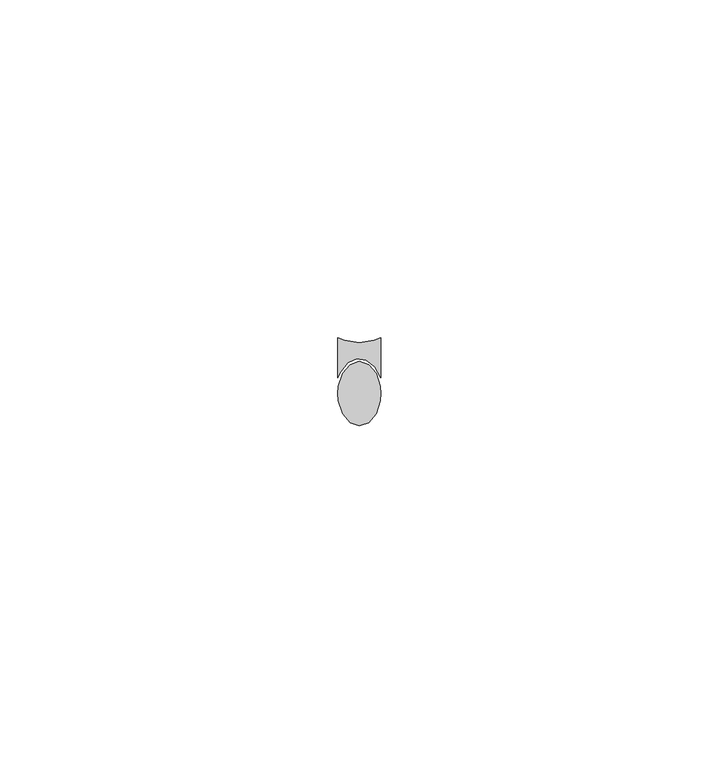
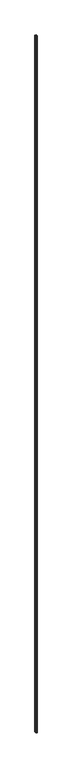
"""IFC4 building model written with IfcOpenShell, lengths in millimetres: proxy geometry, Generic Models 11:Generic Models 1:306267:Generic Models 1:306267 : Generic Models 11:Generic Models 1:306267:300405:Generic Models 1:306267:Generic Models 1:306267 : Generic Models 11:Generic Models 1:306267:300405 : Generic Models 11:Generic Models 1:306267:Generic Models 1:306267 : Generic Models 11:Generic Models 1:306267:300405:3 : Generic Models 11:Generic Models 1:306267:Generic Models 1:306267 : Generic Models 11:Generic Models 1:306267:300405:Generic Models 1:306267:Generic Models 1:306267 : Generic Models 11:Generic Models 1:306267:300405 : Generic Models 11:Generic Models 1:306267:Generic Models 1:306267 : Generic Models 11:Generic Models 1:306267:300405:300182."""

import ifcopenshell
import ifcopenshell.guid

model = None  # the IFC model being written
_history = None  # IfcOwnerHistory: only IFC2X3 demands one
_inside = {}  # id of a spatial element -> (the spatial element, [elements in it])
_under = {}  # id of a project, library or spatial element -> (it, [spatial elements below it])
_declared = {}  # id of a project -> (the project, [libraries it declares])
_typed = {}  # id of a type object -> (the type object, [elements of that type])
_made_of = {}  # id of a material, layer set ... -> (it, [elements and type objects made of it])


def new_model(schema):
    """Start an empty IFC model of exactly this schema.

    Asked for "IFC4X3", IfcOpenShell would pick the latest addendum, in which some entities
    have other attributes; the version numbers below select the first issue.
    IFC2X3 requires an IfcOwnerHistory on every rooted entity: one is made here for all.
    """
    global model, _history
    if schema == "IFC4X3":
        model = ifcopenshell.file(schema_version=(4, 3, 0, 0))
    else:
        model = ifcopenshell.file(schema=schema)
    _inside.clear()
    _under.clear()
    _declared.clear()
    _typed.clear()
    _made_of.clear()
    _history = None
    if model.schema == "IFC2X3":
        org = make("IfcOrganization", Name="unknown")
        user = make(
            "IfcPersonAndOrganization",
            ThePerson=make("IfcPerson", FamilyName="unknown"),
            TheOrganization=org,
        )
        app = make(
            "IfcApplication",
            ApplicationDeveloper=org,
            Version="unknown",
            ApplicationFullName="unknown",
            ApplicationIdentifier="unknown",
        )
        _history = make(
            "IfcOwnerHistory",
            OwningUser=user,
            OwningApplication=app,
            ChangeAction="ADDED",
            CreationDate=0,
        )
    return model


def make(cls, **values):
    """One entity of the class cls with the attributes given. An attribute that is None is left unset."""
    return model.create_entity(
        cls, **{name: value for name, value in values.items() if value is not None}
    )


def rooted(cls, **values):
    """An entity with a GlobalId (a new one), such as an element, a storey or a relation."""
    return make(cls, GlobalId=ifcopenshell.guid.new(), OwnerHistory=_history, **values)


def si_unit(unit_type, name, prefix=None):
    """IfcSIUnit, for example si_unit("LENGTHUNIT", "METRE", prefix="MILLI")."""
    return make("IfcSIUnit", UnitType=unit_type, Prefix=prefix, Name=name)


def assignment(units):
    """IfcUnitAssignment: the units of a project."""
    return None if units is None else make("IfcUnitAssignment", Units=units)


def point(xyz):
    """IfcCartesianPoint."""
    return None if xyz is None else make("IfcCartesianPoint", Coordinates=xyz)


def direction(xyz):
    """IfcDirection."""
    return None if xyz is None else make("IfcDirection", DirectionRatios=xyz)


def frame(location, z_axis=None, x_axis=None):
    """IfcAxis2Placement3D, a coordinate frame: its origin and axes. An axis left out is left unset."""
    return make(
        "IfcAxis2Placement3D",
        Location=point(location),
        Axis=direction(z_axis),
        RefDirection=direction(x_axis),
    )


def origin():
    """The frame at (0, 0, 0) with its axes left unset."""
    return frame((0.0, 0.0, 0.0))


def place(relative_to, where):
    """IfcLocalPlacement: puts the frame where relative to a parent placement (None: the world)."""
    return make(
        "IfcLocalPlacement", PlacementRelTo=relative_to, RelativePlacement=where
    )


def context(
    kind, dimensions, precision=None, world=None, true_north=None, identifier=None
):
    """IfcGeometricRepresentationContext, for example the 3D "Model" context."""
    return make(
        "IfcGeometricRepresentationContext",
        ContextIdentifier=identifier,
        ContextType=kind,
        CoordinateSpaceDimension=dimensions,
        Precision=precision,
        WorldCoordinateSystem=world,
        TrueNorth=true_north,
    )


def project(units=None, contexts=None):
    """IfcProject with its units and contexts."""
    return rooted(
        "IfcProject",
        Name="project",
        RepresentationContexts=contexts,
        UnitsInContext=assignment(units),
    )


def spatial(cls, under=None, at=None, **own):
    """A site, building, storey or space (cls), placed at a placement, below another one or the project."""
    s = rooted(cls, ObjectPlacement=at, **own)
    if under is not None:
        _under.setdefault(under.id(), (under, []))[1].append(s)
    return s


def polyline(points):
    """IfcPolyline through the points."""
    return make("IfcPolyline", Points=[point(p) for p in points])


def outline(outer, holes=None, kind="AREA"):
    """IfcArbitraryClosedProfileDef: a profile drawn as a closed curve; with holes, ...WithVoids."""
    if holes is None:
        return make("IfcArbitraryClosedProfileDef", ProfileType=kind, OuterCurve=outer)
    return make(
        "IfcArbitraryProfileDefWithVoids",
        ProfileType=kind,
        OuterCurve=outer,
        InnerCurves=holes,
    )


def extrude(swept, where, along, depth):
    """IfcExtrudedAreaSolid: the profile swept, set in the frame where, extruded along a direction by depth."""
    return make(
        "IfcExtrudedAreaSolid",
        SweptArea=swept,
        Position=where,
        ExtrudedDirection=direction(along),
        Depth=depth,
    )


def shape(context_of_items, identifier, shape_type, items):
    """IfcShapeRepresentation: the items that make up one representation, for example the "Body"."""
    return make(
        "IfcShapeRepresentation",
        ContextOfItems=context_of_items,
        RepresentationIdentifier=identifier,
        RepresentationType=shape_type,
        Items=items,
    )


def source(mapping_origin, context_of_items, identifier, shape_type, items):
    """IfcRepresentationMap: a shape defined once, which mapped items show again and again."""
    return make(
        "IfcRepresentationMap",
        MappingOrigin=mapping_origin,
        MappedRepresentation=shape(context_of_items, identifier, shape_type, items),
    )


def transform(
    local_origin,
    x_axis=None,
    y_axis=None,
    z_axis=None,
    scale=None,
    scale2=None,
    scale3=None,
    uniform=True,
):
    """IfcCartesianTransformationOperator3D, or its non-uniform kind. x_axis, y_axis, z_axis: its Axis1, 2, 3."""
    if uniform:
        return make(
            "IfcCartesianTransformationOperator3D",
            Axis1=direction(x_axis),
            Axis2=direction(y_axis),
            LocalOrigin=point(local_origin),
            Scale=scale,
            Axis3=direction(z_axis),
        )
    return make(
        "IfcCartesianTransformationOperator3DnonUniform",
        Axis1=direction(x_axis),
        Axis2=direction(y_axis),
        LocalOrigin=point(local_origin),
        Scale=scale,
        Axis3=direction(z_axis),
        Scale2=scale2,
        Scale3=scale3,
    )


def mapped(mapping_source, mapping_target):
    """IfcMappedItem: shows the shape of a source again, moved by a transform."""
    return make(
        "IfcMappedItem", MappingSource=mapping_source, MappingTarget=mapping_target
    )


def made_of(thing, what):
    """Note that an element or type object is made of a material, layer set ...; save() writes the relation."""
    if what is not None:
        _made_of.setdefault(what.id(), (what, []))[1].append(thing)
    return thing


def element(
    cls,
    number,
    at=None,
    inside=None,
    cuts=None,
    type_object=None,
    material=None,
    context=None,
    identifier="Body",
    shape_type=None,
    held_by="IfcProductDefinitionShape",
    body=None,
    shapes=None,
    **own,
):
    """One element of the class cls, such as IfcWall. Its Tag is "e" and its number.

    at: its placement. inside: the storey or other place that contains it. cuts: it is an
    opening in that element (IfcRelVoidsElement). A single representation is given by context,
    identifier, shape_type and body (its items); several are given by shapes. held_by: the class
    of the entity that holds the representations. save() writes the other relations.
    """
    e = rooted(cls, Tag="e%d" % number, ObjectPlacement=at, **own)
    if body is not None:
        shapes = [shape(context, identifier, shape_type, body)]
    if shapes is not None:
        e.Representation = make(held_by, Representations=shapes)
    if inside is not None:
        _inside.setdefault(inside.id(), (inside, []))[1].append(e)
    if cuts is not None:
        rooted(
            "IfcRelVoidsElement", RelatingBuildingElement=cuts, RelatedOpeningElement=e
        )
    if type_object is not None:
        _typed.setdefault(type_object.id(), (type_object, []))[1].append(e)
    return made_of(e, material)


def aggregate(whole, parts):
    """IfcRelAggregates: a whole, such as a stair, and the parts it consists of."""
    return rooted("IfcRelAggregates", RelatingObject=whole, RelatedObjects=parts)


def save(model, path):
    """Write the relations noted so far, then the file.

    IfcRelAggregates (storeys below a building ...), IfcRelContainedInSpatialStructure (elements
    in a storey), IfcRelDefinesByType, IfcRelAssociatesMaterial and IfcRelDeclares: one each for
    every whole, place, type object, material and project.
    """
    for whole, parts in _under.values():
        aggregate(whole, parts)
    for where, things in _inside.values():
        rooted(
            "IfcRelContainedInSpatialStructure",
            RelatedElements=things,
            RelatingStructure=where,
        )
    for kind, things in _typed.values():
        rooted("IfcRelDefinesByType", RelatedObjects=things, RelatingType=kind)
    for what, things in _made_of.values():
        rooted("IfcRelAssociatesMaterial", RelatedObjects=things, RelatingMaterial=what)
    for by, libraries in _declared.values():
        rooted("IfcRelDeclares", RelatingContext=by, RelatedDefinitions=libraries)
    model.write(path)


def generic_models_c62f5399(model_context):
    return source(origin(), model_context, "Body", "SweptSolid", [
        extrude(outline(polyline([(592757.2216431, -579051.613272), (592758.5992239, -579051.1416362), (592759.9768048, -579051.613272), (592761.0815389, -579052.9347661), (592761.6946201, -579054.8443803), (592761.7742239, -579055.9041362), (592761.6946201, -579056.9638922), (592761.0815389, -579058.8735064), (592759.9768048, -579060.1950005), (592758.5992239, -579060.6666362), (592757.2216431, -579060.1950005), (592756.116909, -579058.8735064), (592755.5038278, -579056.9638922), (592755.4242239, -579055.9041362), (592755.5038278, -579054.8443803), (592756.116909, -579052.9347661), (592757.2216431, -579051.613272)])), frame((0.0, 0.0, 31.75), z_axis=(0.0, 0.0, 1.0), x_axis=(1.0, 0.0, 0.0)), (0.0, 0.0, 1.0), 3663.95),
        extrude(outline(polyline([(592760.8084607, -579048.0498252), (592761.7742239, -579047.6724166), (592761.7742239, -579053.5405087), (592760.8914351, -579051.9472919), (592759.650051, -579050.9730869), (592758.2442747, -579050.770299), (592756.894027, -579051.3706525), (592755.8105415, -579052.6802277), (592755.4242239, -579053.5405087), (592755.4242239, -579047.6724166), (592756.3899872, -579048.0498252), (592758.5992239, -579048.3635112), (592760.8084607, -579048.0498252)])), frame((0.0, 0.0, 31.75), z_axis=(0.0, 0.0, 1.0), x_axis=(1.0, 0.0, 0.0)), (0.0, 0.0, 1.0), 3663.95),
    ])


if __name__ == "__main__":
    model = new_model("IFC4")
    model_context = context("Model", 3, world=origin())
    ifc_project = project(units=[si_unit("LENGTHUNIT", "METRE", prefix="MILLI")], contexts=[model_context])
    site = spatial("IfcSite", under=ifc_project)
    building = spatial("IfcBuilding", under=site)
    placement = place(None, origin())
    generic_models_shape = generic_models_c62f5399(model_context)
    element("IfcBuildingElementProxy", 1, Name="Generic Models 11:Generic Models 1:306267:Generic Models 1:306267 : Generic Models 11:Generic Models 1:306267:300405:Generic Models 1:306267:Generic Models 1:306267 : Generic Models 11:Generic Models 1:306267:300405 : Generic Models 11:Generic Models 1:306267:Generic Models 1:306267 : Generic Models 11:Generic Models 1:306267:300405:3 : Generic Models 11:Generic Models 1:306267:Generic Models 1:306267 : Generic Models 11:Generic Models 1:306267:300405:Generic Models 1:306267:Generic Models 1:306267 : Generic Models 11:Generic Models 1:306267:300405 : Generic Models 11:Generic Models 1:306267:Generic Models 1:306267 : Generic Models 11:Generic Models 1:306267:300405:300182", ObjectType="Generic Models 11:Generic Models 1:306267:Generic Models 1:306267 : Generic Models 11:Generic Models 1:306267:300405:Generic Models 1:306267:Generic Models 1:306267 : Generic Models 11:Generic Models 1:306267:300405 : Generic Models 11:Generic Models 1:306267:Generic Models 1:306267 : Generic Models 11:Generic Models 1:306267:300405:3 : Generic Models 11:Generic Models 1:306267:Generic Models 1:306267 : Generic Models 11:Generic Models 1:306267:300405:Generic Models 1:306267:Generic Models 1:306267 : Generic Models 11:Generic Models 1:306267:300405 : Generic Models 11:Generic Models 1:306267:Generic Models 1:306267 : Generic Models 11:Generic Models 1:306267:300405:300182", at=placement, inside=building, context=model_context, shape_type="MappedRepresentation", body=[
        mapped(generic_models_shape, transform((0.0, 0.0, 0.0), x_axis=(1.0, 0.0, 0.0), y_axis=(0.0, 1.0, 0.0), z_axis=(0.0, 0.0, 1.0))),
    ])
    save(model, "model.ifc")

# Revit data of these elements
# Type "Generic Models 11:Generic Models 1:306267:Generic Models 1:306267 : Generic Models 11:Generic Models 1:306267:300405:Generic Models 1:306267:Generic Models 1:306267 : Generic Models 11:Generic Models 1:306267:300405 : Generic Models 11:Generic Models 1:306267:Generic Models 1:306267 : Generic Models 11:Generic Models 1:306267:300405:3 : Generic Models 11:Generic Models 1:306267:Generic Models 1:306267 : Generic Models 11:Generic Models 1:306267:300405:Generic Models 1:306267:Generic Models 1:306267 : Generic Models 11:Generic Models 1:306267:300405 : Generic Models 11:Generic Models 1:306267:Generic Models 1:306267 : Generic Models 11:Generic Models 1:306267:300405:300182"
#   NameOverride = "Generic Models 11:Generic Models 1:306267:Generic Models 1:306267 : Generic Models 11:Generic Models 1:306267:300405:Generic Models 1:306267:Generic Models 1:306267 : Generic Models 11:Generic Models 1:306267:300405 : Generic Models 11:Generic Models 1:306267:Generic Models 1:306267 : Generic Models 11:Generic Models 1:306267:300405:300182"
#   ObjectTypeOverride = "Generic Models 1:306267:Generic Models 1:306267 : Generic Models 11:Generic Models 1:306267:300405 : Generic Models 11:Generic Models 1:306267:Generic Models 1:306267 : Generic Models 11:Generic Models 1:306267:300405"
#   Reference = "Generic Models 1"
#   Tag = "300182"
# Element 1 (IfcBuildingElementProxy, "Generic Models 11:Generic Models 1:306267:Generic Models 1:306267 : Generic Models 11:Generic Models 1:306267:300405:Generic Models 1:306267:Generic Models 1:306267 : Generic Models 11:Generic Models 1:306267:300405 : Generic Models 11:Generic Models 1:306267:Generic Models 1:306267 : Generic Models 11:Generic Models 1:306267:300405:3 : Generic Models 11:Generic Models 1:306267:Generic Models 1:306267 : Generic Models 11:Generic Models 1:306267:300405:Generic Models 1:306267:Generic Models 1:306267 : Generic Models 11:Generic Models 1:306267:300405 : Generic Models 11:Generic Models 1:306267:Generic Models 1:306267 : Generic Models 11:Generic Models 1:306267:300405:300182")
#   Materials on its faces: "SEALANT & BACKER ROD, IF NECESSARY"
# Materials
#   "SEALANT & BACKER ROD, IF NECESSARY": class "Unassigned", colour RGB 120 120 120, transparency 0, Cost = 0
